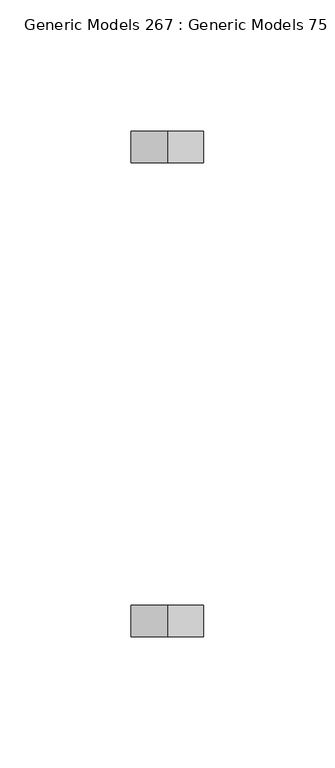
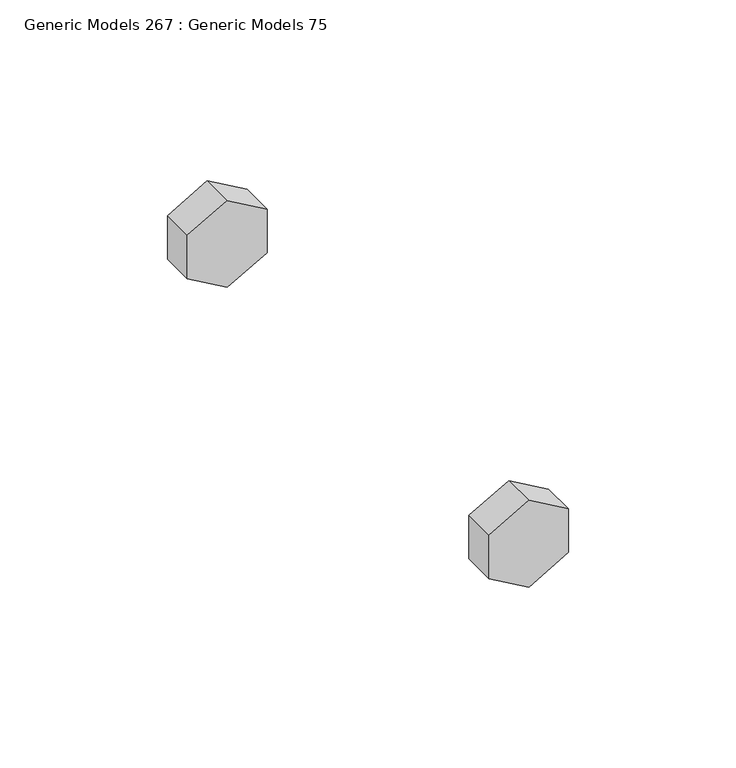
"""IFC4 building model written with IfcOpenShell, lengths in millimetres: proxy geometry, Generic Models 267 : Generic Models 75."""

from ifc_helpers import new_model, si_unit, frame, origin, place, context, project, spatial, polyline, outline, extrude, source, transform, mapped, element, save


def generic_models_267_generic_models_75_ae5ef65d(model_context):
    return source(origin(), model_context, "Body", "SweptSolid", [
        extrude(outline(polyline([(268536.8902933, 31975.9942029), (268521.0537198, 31975.9942029), (268513.135433, 31989.7090778), (268521.0537198, 32003.4239528), (268536.8902933, 32003.4239528), (268544.80858, 31989.7090778), (268536.8902933, 31975.9942029)])), frame((0.0, 30858.4781612, 0.0), z_axis=(0.0, 1.0, 0.0), x_axis=(0.0, 0.0, 1.0)), (0.0, 0.0, 1.0), 11.90625),
        extrude(outline(polyline([(268536.8902933, 31975.9942029), (268521.0537198, 31975.9942029), (268513.135433, 31989.7090778), (268521.0537198, 32003.4239528), (268536.8902933, 32003.4239528), (268544.80858, 31989.7090778), (268536.8902933, 31975.9942029)])), frame((0.0, 30678.2969112, 0.0), z_axis=(0.0, 1.0, 0.0), x_axis=(0.0, 0.0, 1.0)), (0.0, 0.0, 1.0), 11.90625),
    ])


if __name__ == "__main__":
    model = new_model("IFC4")
    model_context = context("Model", 3, world=origin())
    ifc_project = project(units=[si_unit("LENGTHUNIT", "METRE", prefix="MILLI")], contexts=[model_context])
    site = spatial("IfcSite", under=ifc_project)
    building = spatial("IfcBuilding", under=site)
    placement = place(None, origin())
    generic_models_267_generic_models_75_shape = generic_models_267_generic_models_75_ae5ef65d(model_context)
    element("IfcBuildingElementProxy", 1, Name="Generic Models 267 : Generic Models 75", ObjectType="Generic Models 267 : Generic Models 75", at=placement, inside=building, context=model_context, shape_type="MappedRepresentation", body=[
        mapped(generic_models_267_generic_models_75_shape, transform((0.0, 0.0, 0.0), x_axis=(1.0, 0.0, 0.0), y_axis=(0.0, 1.0, 0.0), z_axis=(0.0, 0.0, 1.0))),
    ])
    save(model, "model.ifc")

# Revit data of these elements
# Element 1 (IfcBuildingElementProxy, "Generic Models 267 : Generic Models 75")
#   Materials on its faces: "3/4\" GALV. THRU BOLTS"
# Materials
#   "3/4\" GALV. THRU BOLTS": class "Generic", colour RGB 105 69 171, transparency 0, Cost = 0
